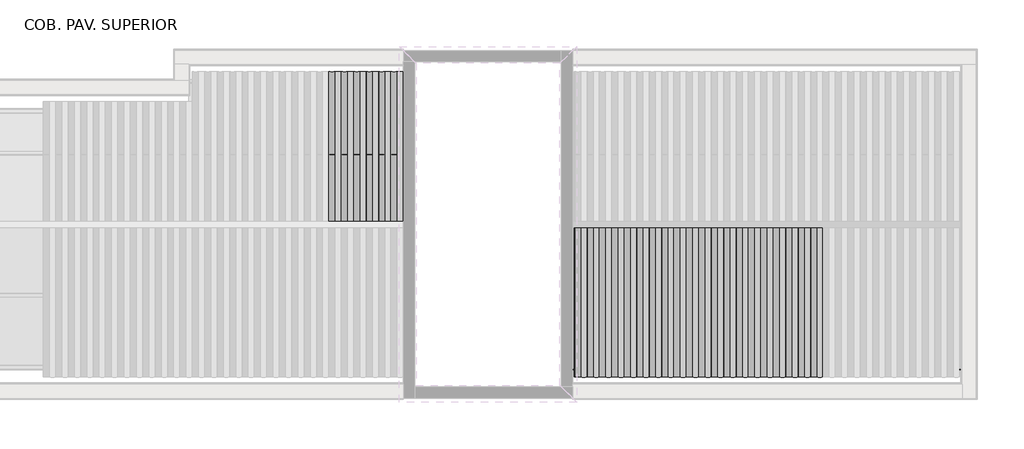
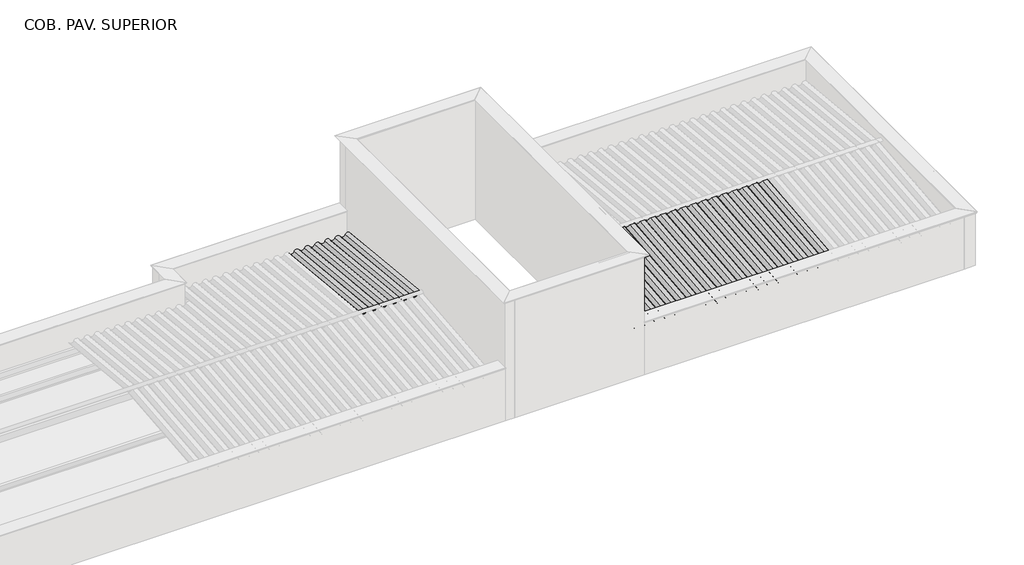
# One storey, part 5 of 7: 36 beams, 9 columns.
"""IFC4 building model written with IfcOpenShell, lengths in millimetres."""

import ifcopenshell
import ifcopenshell.guid

model = None  # the IFC model being written
_history = None  # IfcOwnerHistory: only IFC2X3 demands one
_inside = {}  # id of a spatial element -> (the spatial element, [elements in it])
_under = {}  # id of a project, library or spatial element -> (it, [spatial elements below it])
_declared = {}  # id of a project -> (the project, [libraries it declares])
_typed = {}  # id of a type object -> (the type object, [elements of that type])
_made_of = {}  # id of a material, layer set ... -> (it, [elements and type objects made of it])


def new_model(schema):
    """Start an empty IFC model of exactly this schema.

    Asked for "IFC4X3", IfcOpenShell would pick the latest addendum, in which some entities
    have other attributes; the version numbers below select the first issue.
    IFC2X3 requires an IfcOwnerHistory on every rooted entity: one is made here for all.
    """
    global model, _history
    if schema == "IFC4X3":
        model = ifcopenshell.file(schema_version=(4, 3, 0, 0))
    else:
        model = ifcopenshell.file(schema=schema)
    _inside.clear()
    _under.clear()
    _declared.clear()
    _typed.clear()
    _made_of.clear()
    _history = None
    if model.schema == "IFC2X3":
        org = make("IfcOrganization", Name="unknown")
        user = make(
            "IfcPersonAndOrganization",
            ThePerson=make("IfcPerson", FamilyName="unknown"),
            TheOrganization=org,
        )
        app = make(
            "IfcApplication",
            ApplicationDeveloper=org,
            Version="unknown",
            ApplicationFullName="unknown",
            ApplicationIdentifier="unknown",
        )
        _history = make(
            "IfcOwnerHistory",
            OwningUser=user,
            OwningApplication=app,
            ChangeAction="ADDED",
            CreationDate=0,
        )
    return model


def make(cls, **values):
    """One entity of the class cls with the attributes given. An attribute that is None is left unset."""
    return model.create_entity(
        cls, **{name: value for name, value in values.items() if value is not None}
    )


def rooted(cls, **values):
    """An entity with a GlobalId (a new one), such as an element, a storey or a relation."""
    return make(cls, GlobalId=ifcopenshell.guid.new(), OwnerHistory=_history, **values)


def si_unit(unit_type, name, prefix=None):
    """IfcSIUnit, for example si_unit("LENGTHUNIT", "METRE", prefix="MILLI")."""
    return make("IfcSIUnit", UnitType=unit_type, Prefix=prefix, Name=name)


def assignment(units):
    """IfcUnitAssignment: the units of a project."""
    return None if units is None else make("IfcUnitAssignment", Units=units)


def point(xyz):
    """IfcCartesianPoint."""
    return None if xyz is None else make("IfcCartesianPoint", Coordinates=xyz)


def direction(xyz):
    """IfcDirection."""
    return None if xyz is None else make("IfcDirection", DirectionRatios=xyz)


def frame(location, z_axis=None, x_axis=None):
    """IfcAxis2Placement3D, a coordinate frame: its origin and axes. An axis left out is left unset."""
    return make(
        "IfcAxis2Placement3D",
        Location=point(location),
        Axis=direction(z_axis),
        RefDirection=direction(x_axis),
    )


def frame_2d(location, x_axis=None):
    """IfcAxis2Placement2D, a coordinate frame in the plane: its origin and x axis."""
    return make(
        "IfcAxis2Placement2D", Location=point(location), RefDirection=direction(x_axis)
    )


def origin():
    """The frame at (0, 0, 0) with its axes left unset."""
    return frame((0.0, 0.0, 0.0))


def place(relative_to, where):
    """IfcLocalPlacement: puts the frame where relative to a parent placement (None: the world)."""
    return make(
        "IfcLocalPlacement", PlacementRelTo=relative_to, RelativePlacement=where
    )


def context(
    kind, dimensions, precision=None, world=None, true_north=None, identifier=None
):
    """IfcGeometricRepresentationContext, for example the 3D "Model" context."""
    return make(
        "IfcGeometricRepresentationContext",
        ContextIdentifier=identifier,
        ContextType=kind,
        CoordinateSpaceDimension=dimensions,
        Precision=precision,
        WorldCoordinateSystem=world,
        TrueNorth=true_north,
    )


def project(units=None, contexts=None):
    """IfcProject with its units and contexts."""
    return rooted(
        "IfcProject",
        Name="project",
        RepresentationContexts=contexts,
        UnitsInContext=assignment(units),
    )


def spatial(cls, under=None, at=None, **own):
    """A site, building, storey or space (cls), placed at a placement, below another one or the project."""
    s = rooted(cls, ObjectPlacement=at, **own)
    if under is not None:
        _under.setdefault(under.id(), (under, []))[1].append(s)
    return s


def polyline(points):
    """IfcPolyline through the points."""
    return make("IfcPolyline", Points=[point(p) for p in points])


def circle_curve(where, radius):
    """IfcCircle in the frame where."""
    return make("IfcCircle", Position=where, Radius=radius)


def trimmed(basis, trim1, trim2, sense, master):
    """IfcTrimmedCurve: the piece of a basis curve between two trims."""
    return make(
        "IfcTrimmedCurve",
        BasisCurve=basis,
        Trim1=trim1,
        Trim2=trim2,
        SenseAgreement=sense,
        MasterRepresentation=master,
    )


def segment(curve, same_sense, transition):
    """IfcCompositeCurveSegment."""
    return make(
        "IfcCompositeCurveSegment",
        Transition=transition,
        SameSense=same_sense,
        ParentCurve=curve,
    )


def composite_curve(segments, self_intersect=None):
    """IfcCompositeCurve: segments joined end to end."""
    return make("IfcCompositeCurve", Segments=segments, SelfIntersect=self_intersect)


def outline(outer, holes=None, kind="AREA"):
    """IfcArbitraryClosedProfileDef: a profile drawn as a closed curve; with holes, ...WithVoids."""
    if holes is None:
        return make("IfcArbitraryClosedProfileDef", ProfileType=kind, OuterCurve=outer)
    return make(
        "IfcArbitraryProfileDefWithVoids",
        ProfileType=kind,
        OuterCurve=outer,
        InnerCurves=holes,
    )


def extrude(swept, where, along, depth):
    """IfcExtrudedAreaSolid: the profile swept, set in the frame where, extruded along a direction by depth."""
    return make(
        "IfcExtrudedAreaSolid",
        SweptArea=swept,
        Position=where,
        ExtrudedDirection=direction(along),
        Depth=depth,
    )


def shape(context_of_items, identifier, shape_type, items):
    """IfcShapeRepresentation: the items that make up one representation, for example the "Body"."""
    return make(
        "IfcShapeRepresentation",
        ContextOfItems=context_of_items,
        RepresentationIdentifier=identifier,
        RepresentationType=shape_type,
        Items=items,
    )


def source(mapping_origin, context_of_items, identifier, shape_type, items):
    """IfcRepresentationMap: a shape defined once, which mapped items show again and again."""
    return make(
        "IfcRepresentationMap",
        MappingOrigin=mapping_origin,
        MappedRepresentation=shape(context_of_items, identifier, shape_type, items),
    )


def transform(
    local_origin,
    x_axis=None,
    y_axis=None,
    z_axis=None,
    scale=None,
    scale2=None,
    scale3=None,
    uniform=True,
):
    """IfcCartesianTransformationOperator3D, or its non-uniform kind. x_axis, y_axis, z_axis: its Axis1, 2, 3."""
    if uniform:
        return make(
            "IfcCartesianTransformationOperator3D",
            Axis1=direction(x_axis),
            Axis2=direction(y_axis),
            LocalOrigin=point(local_origin),
            Scale=scale,
            Axis3=direction(z_axis),
        )
    return make(
        "IfcCartesianTransformationOperator3DnonUniform",
        Axis1=direction(x_axis),
        Axis2=direction(y_axis),
        LocalOrigin=point(local_origin),
        Scale=scale,
        Axis3=direction(z_axis),
        Scale2=scale2,
        Scale3=scale3,
    )


def mapped(mapping_source, mapping_target):
    """IfcMappedItem: shows the shape of a source again, moved by a transform."""
    return make(
        "IfcMappedItem", MappingSource=mapping_source, MappingTarget=mapping_target
    )


def made_of(thing, what):
    """Note that an element or type object is made of a material, layer set ...; save() writes the relation."""
    if what is not None:
        _made_of.setdefault(what.id(), (what, []))[1].append(thing)
    return thing


def element(
    cls,
    number,
    at=None,
    inside=None,
    cuts=None,
    type_object=None,
    material=None,
    context=None,
    identifier="Body",
    shape_type=None,
    held_by="IfcProductDefinitionShape",
    body=None,
    shapes=None,
    **own,
):
    """One element of the class cls, such as IfcWall. Its Tag is "e" and its number.

    at: its placement. inside: the storey or other place that contains it. cuts: it is an
    opening in that element (IfcRelVoidsElement). A single representation is given by context,
    identifier, shape_type and body (its items); several are given by shapes. held_by: the class
    of the entity that holds the representations. save() writes the other relations.
    """
    e = rooted(cls, Tag="e%d" % number, ObjectPlacement=at, **own)
    if body is not None:
        shapes = [shape(context, identifier, shape_type, body)]
    if shapes is not None:
        e.Representation = make(held_by, Representations=shapes)
    if inside is not None:
        _inside.setdefault(inside.id(), (inside, []))[1].append(e)
    if cuts is not None:
        rooted(
            "IfcRelVoidsElement", RelatingBuildingElement=cuts, RelatedOpeningElement=e
        )
    if type_object is not None:
        _typed.setdefault(type_object.id(), (type_object, []))[1].append(e)
    return made_of(e, material)


def aggregate(whole, parts):
    """IfcRelAggregates: a whole, such as a stair, and the parts it consists of."""
    return rooted("IfcRelAggregates", RelatingObject=whole, RelatedObjects=parts)


def save(model, path):
    """Write the relations noted so far, then the file.

    IfcRelAggregates (storeys below a building ...), IfcRelContainedInSpatialStructure (elements
    in a storey), IfcRelDefinesByType, IfcRelAssociatesMaterial and IfcRelDeclares: one each for
    every whole, place, type object, material and project.
    """
    for whole, parts in _under.values():
        aggregate(whole, parts)
    for where, things in _inside.values():
        rooted(
            "IfcRelContainedInSpatialStructure",
            RelatedElements=things,
            RelatingStructure=where,
        )
    for kind, things in _typed.values():
        rooted("IfcRelDefinesByType", RelatedObjects=things, RelatingType=kind)
    for what, things in _made_of.values():
        rooted("IfcRelAssociatesMaterial", RelatedObjects=things, RelatingMaterial=what)
    for by, libraries in _declared.values():
        rooted("IfcRelDeclares", RelatingContext=by, RelatedDefinitions=libraries)
    model.write(path)


def column_4db371bd(model_context):
    return source(origin(), model_context, "Body", "SweptSolid", [
        extrude(outline(polyline([(30.0, 80.0), (30.0, -80.0), (-30.0, -80.0), (-30.0, 80.0), (30.0, 80.0)])), frame((0.0, 0.0, 6710.0), z_axis=(0.0, 0.0, 1.0), x_axis=(1.0, 0.0, 0.0)), (0.0, 0.0, 1.0), 660.0),
    ])


def column_e8b88e91(model_context):
    return source(origin(), model_context, "Body", "SweptSolid", [
        extrude(outline(polyline([(30.0, 80.0), (30.0, -80.0), (-30.0, -80.0), (-30.0, 80.0), (30.0, 80.0)])), frame((0.0, 0.0, 6710.0), z_axis=(0.0, 0.0, 1.0), x_axis=(1.0, 0.0, 0.0)), (0.0, 0.0, 1.0), 515.0),
    ])


def column_d0cf395a(model_context):
    return source(origin(), model_context, "Body", "SweptSolid", [
        extrude(outline(polyline([(30.0, 80.0), (30.0, -80.0), (-30.0, -80.0), (-30.0, 80.0), (30.0, 80.0)])), frame((0.0, 0.0, 6710.0), z_axis=(0.0, 0.0, 1.0), x_axis=(1.0, 0.0, 0.0)), (0.0, 0.0, 1.0), 520.0),
    ])


model = new_model("IFC4")

# Units and contexts
model_context = context("Model", 3, world=origin())
ifc_project = project(units=[si_unit("LENGTHUNIT", "METRE", prefix="MILLI")], contexts=[model_context])

# Site, building, storey
site = spatial("IfcSite", under=ifc_project)
building = spatial("IfcBuilding", under=site)
storey = spatial("IfcBuildingStorey", under=building, Name="COB. PAV. SUPERIOR", Elevation=6650.0)

# Beams
placement = place(None, origin())
element("IfcBeam", 1, ObjectType="Madeira de lei : Berço 6x12cm", at=placement, inside=storey, context=model_context, shape_type="SweptSolid", body=[
    extrude(outline(polyline([(-679.2813076, -6319.8711004), (-679.2813076, -6439.8711004), (-2679.2813064, -6439.8711004), (-2679.2813064, -6319.8711004), (-679.2813076, -6319.8711004)])), frame((0.0, 0.0, 6650.0), z_axis=(0.0, 0.0, 1.0), x_axis=(1.0, 0.0, 0.0)), (0.0, 0.0, 1.0), 60.0),
])
element("IfcBeam", 2, ObjectType="Madeira de lei : Berço 6x12cm", at=placement, inside=storey, context=model_context, shape_type="SweptSolid", body=[
    extrude(outline(polyline([(-259.281307, -6319.8711004), (-259.281307, -6439.8711004), (-679.2813064, -6439.8711004), (-679.2813064, -6319.8711004), (-259.281307, -6319.8711004)])), frame((0.0, 0.0, 6650.0), z_axis=(0.0, 0.0, 1.0), x_axis=(1.0, 0.0, 0.0)), (0.0, 0.0, 1.0), 60.0),
])
element("IfcBeam", 3, ObjectType="Madeira de lei : Berço 6x12cm", at=placement, inside=storey, context=model_context, shape_type="SweptSolid", body=[
    extrude(outline(polyline([(5089.718693, -9101.268869), (5089.718693, -9221.268869), (3089.718693, -9221.268869), (3089.718693, -9101.268869), (5089.718693, -9101.268869)])), frame((0.0, 0.0, 6650.0), z_axis=(0.0, 0.0, 1.0), x_axis=(1.0, 0.0, 0.0)), (0.0, 0.0, 1.0), 60.0),
])
element("IfcBeam", 4, ObjectType="Madeira de lei : Berço 6x12cm", at=placement, inside=storey, context=model_context, shape_type="SweptSolid", body=[
    extrude(outline(polyline([(5089.718693, -10521.818869), (5089.718693, -10641.818869), (3089.718693, -10641.818869), (3089.718693, -10521.818869), (5089.718693, -10521.818869)])), frame((0.0, 0.0, 6650.0), z_axis=(0.0, 0.0, 1.0), x_axis=(1.0, 0.0, 0.0)), (0.0, 0.0, 1.0), 60.0),
])
element("IfcBeam", 5, ObjectType="Madeira de lei : Berço 6x12cm", at=placement, inside=storey, context=model_context, shape_type="SweptSolid", body=[
    extrude(outline(polyline([(7089.718693, -9101.268869), (7089.718693, -9221.268869), (5089.718693, -9221.268869), (5089.718693, -9101.268869), (7089.718693, -9101.268869)])), frame((0.0, 0.0, 6650.0), z_axis=(0.0, 0.0, 1.0), x_axis=(1.0, 0.0, 0.0)), (0.0, 0.0, 1.0), 60.0),
])
element("IfcBeam", 6, ObjectType="Madeira de lei : Berço 6x12cm", at=placement, inside=storey, context=model_context, shape_type="SweptSolid", body=[
    extrude(outline(polyline([(7089.718693, -10521.818869), (7089.718693, -10641.818869), (5089.718693, -10641.818869), (5089.718693, -10521.818869), (7089.718693, -10521.818869)])), frame((0.0, 0.0, 6650.0), z_axis=(0.0, 0.0, 1.0), x_axis=(1.0, 0.0, 0.0)), (0.0, 0.0, 1.0), 60.0),
])
element("IfcBeam", 7, ObjectType="Madeira de lei : Berço 6x12cm", at=placement, inside=storey, context=model_context, shape_type="SweptSolid", body=[
    extrude(outline(polyline([(9089.718693, -10521.818869), (9089.718693, -10641.818869), (7089.718693, -10641.818869), (7089.718693, -10521.818869), (9089.718693, -10521.818869)])), frame((0.0, 0.0, 6650.0), z_axis=(0.0, 0.0, 1.0), x_axis=(1.0, 0.0, 0.0)), (0.0, 0.0, 1.0), 60.0),
])
element("IfcBeam", 8, ObjectType="Madeira de lei : Berço 6x12cm", at=placement, inside=storey, context=model_context, shape_type="SweptSolid", body=[
    extrude(outline(polyline([(10729.718693, -10521.818869), (10729.718693, -10641.818869), (9089.718693, -10641.818869), (9089.718693, -10521.818869), (10729.718693, -10521.818869)])), frame((0.0, 0.0, 6650.0), z_axis=(0.0, 0.0, 1.0), x_axis=(1.0, 0.0, 0.0)), (0.0, 0.0, 1.0), 60.0),
])
element("IfcBeam", 9, ObjectType="Madeira de lei : Berço 6x12cm", at=placement, inside=storey, context=model_context, shape_type="SweptSolid", body=[
    extrude(outline(polyline([(-270.281307, -4899.3026908), (-270.281307, -5019.3026908), (-2270.2813064, -5019.3026908), (-2270.2813064, -4899.3026908), (-270.281307, -4899.3026908)])), frame((0.0, 0.0, 6650.0), z_axis=(0.0, 0.0, 1.0), x_axis=(1.0, 0.0, 0.0)), (0.0, 0.0, 1.0), 60.0),
])
element("IfcBeam", 10, ObjectType="Madeira de lei : Berço 6x12cm", at=placement, inside=storey, context=model_context, shape_type="SweptSolid", body=[
    extrude(outline(polyline([(-2270.2813076, -4899.3026908), (-2270.2813076, -5019.3026908), (-4270.281307, -5019.3026908), (-4270.281307, -4899.3026908), (-2270.2813076, -4899.3026908)])), frame((0.0, 0.0, 6650.0), z_axis=(0.0, 0.0, 1.0), x_axis=(1.0, 0.0, 0.0)), (0.0, 0.0, 1.0), 60.0),
])
element("IfcBeam", 11, ObjectType="Telha Ondulada : Fibrocimento", at=placement, inside=storey, context=model_context, shape_type="SweptSolid", body=[
    extrude(outline(composite_curve([segment(trimmed(circle_curve(frame_2d((0.0, 66.7939461)), 66.7939461), [point((29.3501489, 6.7939461))], [point((29.3501489, 126.7939461))], True, "CARTESIAN"), True, "CONTINUOUS"), segment(polyline([(29.3501489, 126.7939461), (31.5472154, 131.2853711)]), True, "CONTINUOUS"), segment(trimmed(circle_curve(frame_2d((0.0, 66.7939461)), 71.7939461), [point((31.5472154, 131.2853711))], [point((31.5472154, 2.3025211))], False, "CARTESIAN"), True, "CONTINUOUS"), segment(trimmed(circle_curve(frame_2d((58.7002978, -53.2060539)), 61.7939461), [point((31.5472154, 2.3025211))], [point((31.5472154, -108.7146289))], True, "CARTESIAN"), True, "CONTINUOUS"), segment(polyline([(31.5472154, -108.7146289), (29.3501489, -113.2060539)]), True, "CONTINUOUS"), segment(trimmed(circle_curve(frame_2d((58.7002978, -53.2060539)), 66.7939461), [point((29.3501489, -113.2060539))], [point((29.3501489, 6.7939461))], False, "CARTESIAN"), True, "CONTINUOUS")], self_intersect=False)), frame((3256.1156257, -10781.9594023, 7394.5315886), z_axis=(0.0, 0.9950371902099894, 0.09950371902099751), x_axis=(0.0, 0.09950371902099751, -0.9950371902099894)), (0.0, 0.0, 1.0), 3017.2387654),
])
element("IfcBeam", 12, ObjectType="Telha Ondulada : Fibrocimento", at=placement, inside=storey, context=model_context, shape_type="SweptSolid", body=[
    extrude(outline(composite_curve([segment(trimmed(circle_curve(frame_2d((0.0, 66.7939461)), 66.7939461), [point((29.3501489, 6.7939461))], [point((29.3501489, 126.7939461))], True, "CARTESIAN"), True, "CONTINUOUS"), segment(polyline([(29.3501489, 126.7939461), (31.5472154, 131.2853711)]), True, "CONTINUOUS"), segment(trimmed(circle_curve(frame_2d((0.0, 66.7939461)), 71.7939461), [point((31.5472154, 131.2853711))], [point((31.5472154, 2.3025211))], False, "CARTESIAN"), True, "CONTINUOUS"), segment(trimmed(circle_curve(frame_2d((58.7002978, -53.2060539)), 61.7939461), [point((31.5472154, 2.3025211))], [point((31.5472154, -108.7146289))], True, "CARTESIAN"), True, "CONTINUOUS"), segment(polyline([(31.5472154, -108.7146289), (29.3501489, -113.2060539)]), True, "CONTINUOUS"), segment(trimmed(circle_curve(frame_2d((58.7002978, -53.2060539)), 66.7939461), [point((29.3501489, -113.2060539))], [point((29.3501489, 6.7939461))], False, "CARTESIAN"), True, "CONTINUOUS")], self_intersect=False)), frame((3500.6156257, -10781.9594023, 7394.5315886), z_axis=(0.0, 0.9950371902099894, 0.09950371902099751), x_axis=(0.0, 0.09950371902099751, -0.9950371902099894)), (0.0, 0.0, 1.0), 3017.2387654),
])
element("IfcBeam", 13, ObjectType="Telha Ondulada : Fibrocimento", at=placement, inside=storey, context=model_context, shape_type="SweptSolid", body=[
    extrude(outline(composite_curve([segment(trimmed(circle_curve(frame_2d((0.0, 66.7939461)), 66.7939461), [point((29.3501489, 6.7939461))], [point((29.3501489, 126.7939461))], True, "CARTESIAN"), True, "CONTINUOUS"), segment(polyline([(29.3501489, 126.7939461), (31.5472154, 131.2853711)]), True, "CONTINUOUS"), segment(trimmed(circle_curve(frame_2d((0.0, 66.7939461)), 71.7939461), [point((31.5472154, 131.2853711))], [point((31.5472154, 2.3025211))], False, "CARTESIAN"), True, "CONTINUOUS"), segment(trimmed(circle_curve(frame_2d((58.7002978, -53.2060539)), 61.7939461), [point((31.5472154, 2.3025211))], [point((31.5472154, -108.7146289))], True, "CARTESIAN"), True, "CONTINUOUS"), segment(polyline([(31.5472154, -108.7146289), (29.3501489, -113.2060539)]), True, "CONTINUOUS"), segment(trimmed(circle_curve(frame_2d((58.7002978, -53.2060539)), 66.7939461), [point((29.3501489, -113.2060539))], [point((29.3501489, 6.7939461))], False, "CARTESIAN"), True, "CONTINUOUS")], self_intersect=False)), frame((3745.1156257, -10781.9594023, 7394.5315886), z_axis=(0.0, 0.9950371902099894, 0.09950371902099751), x_axis=(0.0, 0.09950371902099751, -0.9950371902099894)), (0.0, 0.0, 1.0), 3017.2387654),
])
element("IfcBeam", 14, ObjectType="Telha Ondulada : Fibrocimento", at=placement, inside=storey, context=model_context, shape_type="SweptSolid", body=[
    extrude(outline(composite_curve([segment(trimmed(circle_curve(frame_2d((0.0, 66.7939461)), 66.7939461), [point((29.3501489, 6.7939461))], [point((29.3501489, 126.7939461))], True, "CARTESIAN"), True, "CONTINUOUS"), segment(polyline([(29.3501489, 126.7939461), (31.5472154, 131.2853711)]), True, "CONTINUOUS"), segment(trimmed(circle_curve(frame_2d((0.0, 66.7939461)), 71.7939461), [point((31.5472154, 131.2853711))], [point((31.5472154, 2.3025211))], False, "CARTESIAN"), True, "CONTINUOUS"), segment(trimmed(circle_curve(frame_2d((58.7002978, -53.2060539)), 61.7939461), [point((31.5472154, 2.3025211))], [point((31.5472154, -108.7146289))], True, "CARTESIAN"), True, "CONTINUOUS"), segment(polyline([(31.5472154, -108.7146289), (29.3501489, -113.2060539)]), True, "CONTINUOUS"), segment(trimmed(circle_curve(frame_2d((58.7002978, -53.2060539)), 66.7939461), [point((29.3501489, -113.2060539))], [point((29.3501489, 6.7939461))], False, "CARTESIAN"), True, "CONTINUOUS")], self_intersect=False)), frame((3989.6156257, -10781.9594023, 7394.5315886), z_axis=(0.0, 0.9950371902099894, 0.09950371902099747), x_axis=(0.0, 0.09950371902099747, -0.9950371902099894)), (0.0, 0.0, 1.0), 3017.2387654),
])
element("IfcBeam", 15, ObjectType="Telha Ondulada : Fibrocimento", at=placement, inside=storey, context=model_context, shape_type="SweptSolid", body=[
    extrude(outline(composite_curve([segment(trimmed(circle_curve(frame_2d((0.0, 66.7939461)), 66.7939461), [point((29.3501489, 6.7939461))], [point((29.3501489, 126.7939461))], True, "CARTESIAN"), True, "CONTINUOUS"), segment(polyline([(29.3501489, 126.7939461), (31.5472154, 131.2853711)]), True, "CONTINUOUS"), segment(trimmed(circle_curve(frame_2d((0.0, 66.7939461)), 71.7939461), [point((31.5472154, 131.2853711))], [point((31.5472154, 2.3025211))], False, "CARTESIAN"), True, "CONTINUOUS"), segment(trimmed(circle_curve(frame_2d((58.7002978, -53.2060539)), 61.7939461), [point((31.5472154, 2.3025211))], [point((31.5472154, -108.7146289))], True, "CARTESIAN"), True, "CONTINUOUS"), segment(polyline([(31.5472154, -108.7146289), (29.3501489, -113.2060539)]), True, "CONTINUOUS"), segment(trimmed(circle_curve(frame_2d((58.7002978, -53.2060539)), 66.7939461), [point((29.3501489, -113.2060539))], [point((29.3501489, 6.7939461))], False, "CARTESIAN"), True, "CONTINUOUS")], self_intersect=False)), frame((4234.1156257, -10781.9594023, 7394.5315886), z_axis=(0.0, 0.9950371902099894, 0.09950371902099747), x_axis=(0.0, 0.09950371902099747, -0.9950371902099894)), (0.0, 0.0, 1.0), 3017.2387654),
])
element("IfcBeam", 16, ObjectType="Telha Ondulada : Fibrocimento", at=placement, inside=storey, context=model_context, shape_type="SweptSolid", body=[
    extrude(outline(composite_curve([segment(trimmed(circle_curve(frame_2d((0.0, 66.7939461)), 66.7939461), [point((29.3501489, 6.7939461))], [point((29.3501489, 126.7939461))], True, "CARTESIAN"), True, "CONTINUOUS"), segment(polyline([(29.3501489, 126.7939461), (31.5472154, 131.2853711)]), True, "CONTINUOUS"), segment(trimmed(circle_curve(frame_2d((0.0, 66.7939461)), 71.7939461), [point((31.5472154, 131.2853711))], [point((31.5472154, 2.3025211))], False, "CARTESIAN"), True, "CONTINUOUS"), segment(trimmed(circle_curve(frame_2d((58.7002978, -53.2060539)), 61.7939461), [point((31.5472154, 2.3025211))], [point((31.5472154, -108.7146289))], True, "CARTESIAN"), True, "CONTINUOUS"), segment(polyline([(31.5472154, -108.7146289), (29.3501489, -113.2060539)]), True, "CONTINUOUS"), segment(trimmed(circle_curve(frame_2d((58.7002978, -53.2060539)), 66.7939461), [point((29.3501489, -113.2060539))], [point((29.3501489, 6.7939461))], False, "CARTESIAN"), True, "CONTINUOUS")], self_intersect=False)), frame((4478.6156257, -10781.9594023, 7394.5315886), z_axis=(0.0, 0.9950371902099894, 0.09950371902099744), x_axis=(0.0, 0.09950371902099744, -0.9950371902099894)), (0.0, 0.0, 1.0), 3017.2387654),
])
element("IfcBeam", 17, ObjectType="Telha Ondulada : Fibrocimento", at=placement, inside=storey, context=model_context, shape_type="SweptSolid", body=[
    extrude(outline(composite_curve([segment(trimmed(circle_curve(frame_2d((0.0, 66.7939461)), 66.7939461), [point((29.3501489, 6.7939461))], [point((29.3501489, 126.7939461))], True, "CARTESIAN"), True, "CONTINUOUS"), segment(polyline([(29.3501489, 126.7939461), (31.5472154, 131.2853711)]), True, "CONTINUOUS"), segment(trimmed(circle_curve(frame_2d((0.0, 66.7939461)), 71.7939461), [point((31.5472154, 131.2853711))], [point((31.5472154, 2.3025211))], False, "CARTESIAN"), True, "CONTINUOUS"), segment(trimmed(circle_curve(frame_2d((58.7002978, -53.2060539)), 61.7939461), [point((31.5472154, 2.3025211))], [point((31.5472154, -108.7146289))], True, "CARTESIAN"), True, "CONTINUOUS"), segment(polyline([(31.5472154, -108.7146289), (29.3501489, -113.2060539)]), True, "CONTINUOUS"), segment(trimmed(circle_curve(frame_2d((58.7002978, -53.2060539)), 66.7939461), [point((29.3501489, -113.2060539))], [point((29.3501489, 6.7939461))], False, "CARTESIAN"), True, "CONTINUOUS")], self_intersect=False)), frame((4723.1156257, -10781.9594023, 7394.5315886), z_axis=(0.0, 0.9950371902099894, 0.09950371902099751), x_axis=(0.0, 0.09950371902099751, -0.9950371902099894)), (0.0, 0.0, 1.0), 3017.2387654),
])
element("IfcBeam", 18, ObjectType="Telha Ondulada : Fibrocimento", at=placement, inside=storey, context=model_context, shape_type="SweptSolid", body=[
    extrude(outline(composite_curve([segment(trimmed(circle_curve(frame_2d((0.0, 66.7939461)), 66.7939461), [point((29.3501489, 6.7939461))], [point((29.3501489, 126.7939461))], True, "CARTESIAN"), True, "CONTINUOUS"), segment(polyline([(29.3501489, 126.7939461), (31.5472154, 131.2853711)]), True, "CONTINUOUS"), segment(trimmed(circle_curve(frame_2d((0.0, 66.7939461)), 71.7939461), [point((31.5472154, 131.2853711))], [point((31.5472154, 2.3025211))], False, "CARTESIAN"), True, "CONTINUOUS"), segment(trimmed(circle_curve(frame_2d((58.7002978, -53.2060539)), 61.7939461), [point((31.5472154, 2.3025211))], [point((31.5472154, -108.7146289))], True, "CARTESIAN"), True, "CONTINUOUS"), segment(polyline([(31.5472154, -108.7146289), (29.3501489, -113.2060539)]), True, "CONTINUOUS"), segment(trimmed(circle_curve(frame_2d((58.7002978, -53.2060539)), 66.7939461), [point((29.3501489, -113.2060539))], [point((29.3501489, 6.7939461))], False, "CARTESIAN"), True, "CONTINUOUS")], self_intersect=False)), frame((4967.6156257, -10781.9594023, 7394.5315886), z_axis=(0.0, 0.9950371902099894, 0.09950371902099751), x_axis=(0.0, 0.09950371902099751, -0.9950371902099894)), (0.0, 0.0, 1.0), 3017.2387654),
])
element("IfcBeam", 19, ObjectType="Telha Ondulada : Fibrocimento", at=placement, inside=storey, context=model_context, shape_type="SweptSolid", body=[
    extrude(outline(composite_curve([segment(trimmed(circle_curve(frame_2d((0.0, 66.7939461)), 66.7939461), [point((29.3501489, 6.7939461))], [point((29.3501489, 126.7939461))], True, "CARTESIAN"), True, "CONTINUOUS"), segment(polyline([(29.3501489, 126.7939461), (31.5472154, 131.2853711)]), True, "CONTINUOUS"), segment(trimmed(circle_curve(frame_2d((0.0, 66.7939461)), 71.7939461), [point((31.5472154, 131.2853711))], [point((31.5472154, 2.3025211))], False, "CARTESIAN"), True, "CONTINUOUS"), segment(trimmed(circle_curve(frame_2d((58.7002978, -53.2060539)), 61.7939461), [point((31.5472154, 2.3025211))], [point((31.5472154, -108.7146289))], True, "CARTESIAN"), True, "CONTINUOUS"), segment(polyline([(31.5472154, -108.7146289), (29.3501489, -113.2060539)]), True, "CONTINUOUS"), segment(trimmed(circle_curve(frame_2d((58.7002978, -53.2060539)), 66.7939461), [point((29.3501489, -113.2060539))], [point((29.3501489, 6.7939461))], False, "CARTESIAN"), True, "CONTINUOUS")], self_intersect=False)), frame((5212.1156257, -10781.9594023, 7394.5315886), z_axis=(0.0, 0.9950371902099894, 0.09950371902099751), x_axis=(0.0, 0.09950371902099751, -0.9950371902099894)), (0.0, 0.0, 1.0), 3017.2387654),
])
element("IfcBeam", 20, ObjectType="Telha Ondulada : Fibrocimento", at=placement, inside=storey, context=model_context, shape_type="SweptSolid", body=[
    extrude(outline(composite_curve([segment(trimmed(circle_curve(frame_2d((0.0, 66.7939461)), 66.7939461), [point((29.3501489, 6.7939461))], [point((29.3501489, 126.7939461))], True, "CARTESIAN"), True, "CONTINUOUS"), segment(polyline([(29.3501489, 126.7939461), (31.5472154, 131.2853711)]), True, "CONTINUOUS"), segment(trimmed(circle_curve(frame_2d((0.0, 66.7939461)), 71.7939461), [point((31.5472154, 131.2853711))], [point((31.5472154, 2.3025211))], False, "CARTESIAN"), True, "CONTINUOUS"), segment(trimmed(circle_curve(frame_2d((58.7002978, -53.2060539)), 61.7939461), [point((31.5472154, 2.3025211))], [point((31.5472154, -108.7146289))], True, "CARTESIAN"), True, "CONTINUOUS"), segment(polyline([(31.5472154, -108.7146289), (29.3501489, -113.2060539)]), True, "CONTINUOUS"), segment(trimmed(circle_curve(frame_2d((58.7002978, -53.2060539)), 66.7939461), [point((29.3501489, -113.2060539))], [point((29.3501489, 6.7939461))], False, "CARTESIAN"), True, "CONTINUOUS")], self_intersect=False)), frame((5456.6156257, -10781.9594023, 7394.5315886), z_axis=(0.0, 0.9950371902099894, 0.09950371902099751), x_axis=(0.0, 0.09950371902099751, -0.9950371902099894)), (0.0, 0.0, 1.0), 3017.2387654),
])
element("IfcBeam", 21, ObjectType="Telha Ondulada : Fibrocimento", at=placement, inside=storey, context=model_context, shape_type="SweptSolid", body=[
    extrude(outline(composite_curve([segment(trimmed(circle_curve(frame_2d((0.0, 66.7939461)), 66.7939461), [point((29.3501489, 6.7939461))], [point((29.3501489, 126.7939461))], True, "CARTESIAN"), True, "CONTINUOUS"), segment(polyline([(29.3501489, 126.7939461), (31.5472154, 131.2853711)]), True, "CONTINUOUS"), segment(trimmed(circle_curve(frame_2d((0.0, 66.7939461)), 71.7939461), [point((31.5472154, 131.2853711))], [point((31.5472154, 2.3025211))], False, "CARTESIAN"), True, "CONTINUOUS"), segment(trimmed(circle_curve(frame_2d((58.7002978, -53.2060539)), 61.7939461), [point((31.5472154, 2.3025211))], [point((31.5472154, -108.7146289))], True, "CARTESIAN"), True, "CONTINUOUS"), segment(polyline([(31.5472154, -108.7146289), (29.3501489, -113.2060539)]), True, "CONTINUOUS"), segment(trimmed(circle_curve(frame_2d((58.7002978, -53.2060539)), 66.7939461), [point((29.3501489, -113.2060539))], [point((29.3501489, 6.7939461))], False, "CARTESIAN"), True, "CONTINUOUS")], self_intersect=False)), frame((5701.1156257, -10781.9594023, 7394.5315886), z_axis=(0.0, 0.9950371902099894, 0.09950371902099747), x_axis=(0.0, 0.09950371902099747, -0.9950371902099894)), (0.0, 0.0, 1.0), 3017.2387654),
])
element("IfcBeam", 22, ObjectType="Telha Ondulada : Fibrocimento", at=placement, inside=storey, context=model_context, shape_type="SweptSolid", body=[
    extrude(outline(composite_curve([segment(trimmed(circle_curve(frame_2d((0.0, 66.7939461)), 66.7939461), [point((29.3501489, 6.7939461))], [point((29.3501489, 126.7939461))], True, "CARTESIAN"), True, "CONTINUOUS"), segment(polyline([(29.3501489, 126.7939461), (31.5472154, 131.2853711)]), True, "CONTINUOUS"), segment(trimmed(circle_curve(frame_2d((0.0, 66.7939461)), 71.7939461), [point((31.5472154, 131.2853711))], [point((31.5472154, 2.3025211))], False, "CARTESIAN"), True, "CONTINUOUS"), segment(trimmed(circle_curve(frame_2d((58.7002978, -53.2060539)), 61.7939461), [point((31.5472154, 2.3025211))], [point((31.5472154, -108.7146289))], True, "CARTESIAN"), True, "CONTINUOUS"), segment(polyline([(31.5472154, -108.7146289), (29.3501489, -113.2060539)]), True, "CONTINUOUS"), segment(trimmed(circle_curve(frame_2d((58.7002978, -53.2060539)), 66.7939461), [point((29.3501489, -113.2060539))], [point((29.3501489, 6.7939461))], False, "CARTESIAN"), True, "CONTINUOUS")], self_intersect=False)), frame((5945.6156257, -10781.9594023, 7394.5315886), z_axis=(0.0, 0.9950371902099894, 0.09950371902099751), x_axis=(0.0, 0.09950371902099751, -0.9950371902099894)), (0.0, 0.0, 1.0), 3017.2387654),
])
element("IfcBeam", 23, ObjectType="Telha Ondulada : Fibrocimento", at=placement, inside=storey, context=model_context, shape_type="SweptSolid", body=[
    extrude(outline(composite_curve([segment(trimmed(circle_curve(frame_2d((0.0, 66.7939461)), 66.7939461), [point((29.3501489, 6.7939461))], [point((29.3501489, 126.7939461))], True, "CARTESIAN"), True, "CONTINUOUS"), segment(polyline([(29.3501489, 126.7939461), (31.5472154, 131.2853711)]), True, "CONTINUOUS"), segment(trimmed(circle_curve(frame_2d((0.0, 66.7939461)), 71.7939461), [point((31.5472154, 131.2853711))], [point((31.5472154, 2.3025211))], False, "CARTESIAN"), True, "CONTINUOUS"), segment(trimmed(circle_curve(frame_2d((58.7002978, -53.2060539)), 61.7939461), [point((31.5472154, 2.3025211))], [point((31.5472154, -108.7146289))], True, "CARTESIAN"), True, "CONTINUOUS"), segment(polyline([(31.5472154, -108.7146289), (29.3501489, -113.2060539)]), True, "CONTINUOUS"), segment(trimmed(circle_curve(frame_2d((58.7002978, -53.2060539)), 66.7939461), [point((29.3501489, -113.2060539))], [point((29.3501489, 6.7939461))], False, "CARTESIAN"), True, "CONTINUOUS")], self_intersect=False)), frame((6190.1156257, -10781.9594023, 7394.5315886), z_axis=(0.0, 0.9950371902099894, 0.09950371902099754), x_axis=(0.0, 0.09950371902099754, -0.9950371902099894)), (0.0, 0.0, 1.0), 3017.2387654),
])
element("IfcBeam", 24, ObjectType="Telha Ondulada : Fibrocimento", at=placement, inside=storey, context=model_context, shape_type="SweptSolid", body=[
    extrude(outline(composite_curve([segment(trimmed(circle_curve(frame_2d((0.0, 66.7939461)), 66.7939461), [point((29.3501489, 6.7939461))], [point((29.3501489, 126.7939461))], True, "CARTESIAN"), True, "CONTINUOUS"), segment(polyline([(29.3501489, 126.7939461), (31.5472154, 131.2853711)]), True, "CONTINUOUS"), segment(trimmed(circle_curve(frame_2d((0.0, 66.7939461)), 71.7939461), [point((31.5472154, 131.2853711))], [point((31.5472154, 2.3025211))], False, "CARTESIAN"), True, "CONTINUOUS"), segment(trimmed(circle_curve(frame_2d((58.7002978, -53.2060539)), 61.7939461), [point((31.5472154, 2.3025211))], [point((31.5472154, -108.7146289))], True, "CARTESIAN"), True, "CONTINUOUS"), segment(polyline([(31.5472154, -108.7146289), (29.3501489, -113.2060539)]), True, "CONTINUOUS"), segment(trimmed(circle_curve(frame_2d((58.7002978, -53.2060539)), 66.7939461), [point((29.3501489, -113.2060539))], [point((29.3501489, 6.7939461))], False, "CARTESIAN"), True, "CONTINUOUS")], self_intersect=False)), frame((6434.6156257, -10781.9594023, 7394.5315886), z_axis=(0.0, 0.9950371902099894, 0.09950371902099751), x_axis=(0.0, 0.09950371902099751, -0.9950371902099894)), (0.0, 0.0, 1.0), 3017.2387654),
])
element("IfcBeam", 25, ObjectType="Telha Ondulada : Fibrocimento", at=placement, inside=storey, context=model_context, shape_type="SweptSolid", body=[
    extrude(outline(composite_curve([segment(trimmed(circle_curve(frame_2d((0.0, 66.7939461)), 66.7939461), [point((29.3501489, 6.7939461))], [point((29.3501489, 126.7939461))], True, "CARTESIAN"), True, "CONTINUOUS"), segment(polyline([(29.3501489, 126.7939461), (31.5472154, 131.2853711)]), True, "CONTINUOUS"), segment(trimmed(circle_curve(frame_2d((0.0, 66.7939461)), 71.7939461), [point((31.5472154, 131.2853711))], [point((31.5472154, 2.3025211))], False, "CARTESIAN"), True, "CONTINUOUS"), segment(trimmed(circle_curve(frame_2d((58.7002978, -53.2060539)), 61.7939461), [point((31.5472154, 2.3025211))], [point((31.5472154, -108.7146289))], True, "CARTESIAN"), True, "CONTINUOUS"), segment(polyline([(31.5472154, -108.7146289), (29.3501489, -113.2060539)]), True, "CONTINUOUS"), segment(trimmed(circle_curve(frame_2d((58.7002978, -53.2060539)), 66.7939461), [point((29.3501489, -113.2060539))], [point((29.3501489, 6.7939461))], False, "CARTESIAN"), True, "CONTINUOUS")], self_intersect=False)), frame((6679.1156257, -10781.9594023, 7394.5315886), z_axis=(0.0, 0.9950371902099894, 0.09950371902099751), x_axis=(0.0, 0.09950371902099751, -0.9950371902099894)), (0.0, 0.0, 1.0), 3017.2387654),
])
element("IfcBeam", 26, ObjectType="Telha Ondulada : Fibrocimento", at=placement, inside=storey, context=model_context, shape_type="SweptSolid", body=[
    extrude(outline(composite_curve([segment(trimmed(circle_curve(frame_2d((0.0, 66.7939461)), 66.7939461), [point((29.3501489, 6.7939461))], [point((29.3501489, 126.7939461))], True, "CARTESIAN"), True, "CONTINUOUS"), segment(polyline([(29.3501489, 126.7939461), (31.5472154, 131.2853711)]), True, "CONTINUOUS"), segment(trimmed(circle_curve(frame_2d((0.0, 66.7939461)), 71.7939461), [point((31.5472154, 131.2853711))], [point((31.5472154, 2.3025211))], False, "CARTESIAN"), True, "CONTINUOUS"), segment(trimmed(circle_curve(frame_2d((58.7002978, -53.2060539)), 61.7939461), [point((31.5472154, 2.3025211))], [point((31.5472154, -108.7146289))], True, "CARTESIAN"), True, "CONTINUOUS"), segment(polyline([(31.5472154, -108.7146289), (29.3501489, -113.2060539)]), True, "CONTINUOUS"), segment(trimmed(circle_curve(frame_2d((58.7002978, -53.2060539)), 66.7939461), [point((29.3501489, -113.2060539))], [point((29.3501489, 6.7939461))], False, "CARTESIAN"), True, "CONTINUOUS")], self_intersect=False)), frame((6923.6156257, -10781.9594023, 7394.5315886), z_axis=(0.0, 0.9950371902099894, 0.09950371902099751), x_axis=(0.0, 0.09950371902099751, -0.9950371902099894)), (0.0, 0.0, 1.0), 3017.2387654),
])
element("IfcBeam", 27, ObjectType="Telha Ondulada : Fibrocimento", at=placement, inside=storey, context=model_context, shape_type="SweptSolid", body=[
    extrude(outline(composite_curve([segment(trimmed(circle_curve(frame_2d((0.0, 66.7939461)), 66.7939461), [point((29.3501489, 6.7939461))], [point((29.3501489, 126.7939461))], True, "CARTESIAN"), True, "CONTINUOUS"), segment(polyline([(29.3501489, 126.7939461), (31.5472154, 131.2853711)]), True, "CONTINUOUS"), segment(trimmed(circle_curve(frame_2d((0.0, 66.7939461)), 71.7939461), [point((31.5472154, 131.2853711))], [point((31.5472154, 2.3025211))], False, "CARTESIAN"), True, "CONTINUOUS"), segment(trimmed(circle_curve(frame_2d((58.7002978, -53.2060539)), 61.7939461), [point((31.5472154, 2.3025211))], [point((31.5472154, -108.7146289))], True, "CARTESIAN"), True, "CONTINUOUS"), segment(polyline([(31.5472154, -108.7146289), (29.3501489, -113.2060539)]), True, "CONTINUOUS"), segment(trimmed(circle_curve(frame_2d((58.7002978, -53.2060539)), 66.7939461), [point((29.3501489, -113.2060539))], [point((29.3501489, 6.7939461))], False, "CARTESIAN"), True, "CONTINUOUS")], self_intersect=False)), frame((7168.1156257, -10781.9594023, 7394.5315886), z_axis=(0.0, 0.9950371902099894, 0.09950371902099751), x_axis=(0.0, 0.09950371902099751, -0.9950371902099894)), (0.0, 0.0, 1.0), 3017.2387654),
])
element("IfcBeam", 28, ObjectType="Telha Ondulada : Fibrocimento", at=placement, inside=storey, context=model_context, shape_type="SweptSolid", body=[
    extrude(outline(composite_curve([segment(trimmed(circle_curve(frame_2d((0.0, 66.7939461)), 66.7939461), [point((29.3501489, 6.7939461))], [point((29.3501489, 126.7939461))], True, "CARTESIAN"), True, "CONTINUOUS"), segment(polyline([(29.3501489, 126.7939461), (31.5472154, 131.2853711)]), True, "CONTINUOUS"), segment(trimmed(circle_curve(frame_2d((0.0, 66.7939461)), 71.7939461), [point((31.5472154, 131.2853711))], [point((31.5472154, 2.3025211))], False, "CARTESIAN"), True, "CONTINUOUS"), segment(trimmed(circle_curve(frame_2d((58.7002978, -53.2060539)), 61.7939461), [point((31.5472154, 2.3025211))], [point((31.5472154, -108.7146289))], True, "CARTESIAN"), True, "CONTINUOUS"), segment(polyline([(31.5472154, -108.7146289), (29.3501489, -113.2060539)]), True, "CONTINUOUS"), segment(trimmed(circle_curve(frame_2d((58.7002978, -53.2060539)), 66.7939461), [point((29.3501489, -113.2060539))], [point((29.3501489, 6.7939461))], False, "CARTESIAN"), True, "CONTINUOUS")], self_intersect=False)), frame((7412.6156257, -10781.9594023, 7394.5315886), z_axis=(0.0, 0.9950371902099894, 0.09950371902099747), x_axis=(0.0, 0.09950371902099747, -0.9950371902099894)), (0.0, 0.0, 1.0), 3017.2387654),
])
element("IfcBeam", 29, ObjectType="Telha Ondulada : Fibrocimento", at=placement, inside=storey, context=model_context, shape_type="SweptSolid", body=[
    extrude(outline(composite_curve([segment(trimmed(circle_curve(frame_2d((0.0, 66.7939461)), 66.7939461), [point((29.3501489, 6.7939461))], [point((29.3501489, 126.7939461))], True, "CARTESIAN"), True, "CONTINUOUS"), segment(polyline([(29.3501489, 126.7939461), (31.5472154, 131.2853711)]), True, "CONTINUOUS"), segment(trimmed(circle_curve(frame_2d((0.0, 66.7939461)), 71.7939461), [point((31.5472154, 131.2853711))], [point((31.5472154, 2.3025211))], False, "CARTESIAN"), True, "CONTINUOUS"), segment(trimmed(circle_curve(frame_2d((58.7002978, -53.2060539)), 61.7939461), [point((31.5472154, 2.3025211))], [point((31.5472154, -108.7146289))], True, "CARTESIAN"), True, "CONTINUOUS"), segment(polyline([(31.5472154, -108.7146289), (29.3501489, -113.2060539)]), True, "CONTINUOUS"), segment(trimmed(circle_curve(frame_2d((58.7002978, -53.2060539)), 66.7939461), [point((29.3501489, -113.2060539))], [point((29.3501489, 6.7939461))], False, "CARTESIAN"), True, "CONTINUOUS")], self_intersect=False)), frame((7657.1156257, -10781.9594023, 7394.5315886), z_axis=(0.0, 0.9950371902099894, 0.09950371902099747), x_axis=(0.0, 0.09950371902099747, -0.9950371902099894)), (0.0, 0.0, 1.0), 3017.2387654),
])
element("IfcBeam", 30, ObjectType="Telha Ondulada : Fibrocimento", at=placement, inside=storey, context=model_context, shape_type="SweptSolid", body=[
    extrude(outline(composite_curve([segment(trimmed(circle_curve(frame_2d((0.0, 66.7939461)), 66.7939461), [point((29.3501489, 6.7939461))], [point((29.3501489, 126.7939461))], True, "CARTESIAN"), True, "CONTINUOUS"), segment(polyline([(29.3501489, 126.7939461), (31.5472154, 131.2853711)]), True, "CONTINUOUS"), segment(trimmed(circle_curve(frame_2d((0.0, 66.7939461)), 71.7939461), [point((31.5472154, 131.2853711))], [point((31.5472154, 2.3025211))], False, "CARTESIAN"), True, "CONTINUOUS"), segment(trimmed(circle_curve(frame_2d((58.7002978, -53.2060539)), 61.7939461), [point((31.5472154, 2.3025211))], [point((31.5472154, -108.7146289))], True, "CARTESIAN"), True, "CONTINUOUS"), segment(polyline([(31.5472154, -108.7146289), (29.3501489, -113.2060539)]), True, "CONTINUOUS"), segment(trimmed(circle_curve(frame_2d((58.7002978, -53.2060539)), 66.7939461), [point((29.3501489, -113.2060539))], [point((29.3501489, 6.7939461))], False, "CARTESIAN"), True, "CONTINUOUS")], self_intersect=False)), frame((7901.6156257, -10781.9594023, 7394.5315886), z_axis=(0.0, 0.9950371902099894, 0.09950371902099751), x_axis=(0.0, 0.09950371902099751, -0.9950371902099894)), (0.0, 0.0, 1.0), 3017.2387654),
])
element("IfcBeam", 31, ObjectType="Telha Ondulada : Fibrocimento", at=placement, inside=storey, context=model_context, shape_type="SweptSolid", body=[
    extrude(outline(composite_curve([segment(trimmed(circle_curve(frame_2d((-58.7002978, -53.2060539)), 66.7939461), [point((-29.3501489, 6.7939461))], [point((-29.3501489, -113.2060539))], False, "CARTESIAN"), True, "CONTINUOUS"), segment(polyline([(-29.3501489, -113.2060539), (-31.5472154, -108.7146289)]), True, "CONTINUOUS"), segment(trimmed(circle_curve(frame_2d((-58.7002978, -53.2060539)), 61.7939461), [point((-31.5472154, -108.7146289))], [point((-31.5472154, 2.3025211))], True, "CARTESIAN"), True, "CONTINUOUS"), segment(trimmed(circle_curve(frame_2d((0.0, 66.7939461)), 71.7939461), [point((-31.5472154, 2.3025211))], [point((-31.5472154, 131.2853711))], False, "CARTESIAN"), True, "CONTINUOUS"), segment(polyline([(-31.5472154, 131.2853711), (-29.3501489, 126.7939461)]), True, "CONTINUOUS"), segment(trimmed(circle_curve(frame_2d((0.0, 66.7939461)), 66.7939461), [point((-29.3501489, 126.7939461))], [point((-29.3501489, 6.7939461))], True, "CARTESIAN"), True, "CONTINUOUS")], self_intersect=False)), frame((-1582.8843743, -4759.1805671, 7394.5315886), z_axis=(0.0, -0.9950371902099893, 0.0995037190209978), x_axis=(0.0, 0.0995037190209978, 0.9950371902099893)), (0.0, 0.0, 1.0), 3017.2295147),
])
element("IfcBeam", 32, ObjectType="Telha Ondulada : Fibrocimento", at=placement, inside=storey, context=model_context, shape_type="SweptSolid", body=[
    extrude(outline(composite_curve([segment(trimmed(circle_curve(frame_2d((-58.7002978, -53.2060539)), 66.7939461), [point((-29.3501489, 6.7939461))], [point((-29.3501489, -113.2060539))], False, "CARTESIAN"), True, "CONTINUOUS"), segment(polyline([(-29.3501489, -113.2060539), (-31.5472154, -108.7146289)]), True, "CONTINUOUS"), segment(trimmed(circle_curve(frame_2d((-58.7002978, -53.2060539)), 61.7939461), [point((-31.5472154, -108.7146289))], [point((-31.5472154, 2.3025211))], True, "CARTESIAN"), True, "CONTINUOUS"), segment(trimmed(circle_curve(frame_2d((0.0, 66.7939461)), 71.7939461), [point((-31.5472154, 2.3025211))], [point((-31.5472154, 131.2853711))], False, "CARTESIAN"), True, "CONTINUOUS"), segment(polyline([(-31.5472154, 131.2853711), (-29.3501489, 126.7939461)]), True, "CONTINUOUS"), segment(trimmed(circle_curve(frame_2d((0.0, 66.7939461)), 66.7939461), [point((-29.3501489, 126.7939461))], [point((-29.3501489, 6.7939461))], True, "CARTESIAN"), True, "CONTINUOUS")], self_intersect=False)), frame((-1338.3843743, -4759.1805671, 7394.5315886), z_axis=(0.0, -0.9950371902099893, 0.09950371902099783), x_axis=(0.0, 0.09950371902099783, 0.9950371902099893)), (0.0, 0.0, 1.0), 3017.2295147),
])
element("IfcBeam", 33, ObjectType="Telha Ondulada : Fibrocimento", at=placement, inside=storey, context=model_context, shape_type="SweptSolid", body=[
    extrude(outline(composite_curve([segment(trimmed(circle_curve(frame_2d((-58.7002978, -53.2060539)), 66.7939461), [point((-29.3501489, 6.7939461))], [point((-29.3501489, -113.2060539))], False, "CARTESIAN"), True, "CONTINUOUS"), segment(polyline([(-29.3501489, -113.2060539), (-31.5472154, -108.7146289)]), True, "CONTINUOUS"), segment(trimmed(circle_curve(frame_2d((-58.7002978, -53.2060539)), 61.7939461), [point((-31.5472154, -108.7146289))], [point((-31.5472154, 2.3025211))], True, "CARTESIAN"), True, "CONTINUOUS"), segment(trimmed(circle_curve(frame_2d((0.0, 66.7939461)), 71.7939461), [point((-31.5472154, 2.3025211))], [point((-31.5472154, 131.2853711))], False, "CARTESIAN"), True, "CONTINUOUS"), segment(polyline([(-31.5472154, 131.2853711), (-29.3501489, 126.7939461)]), True, "CONTINUOUS"), segment(trimmed(circle_curve(frame_2d((0.0, 66.7939461)), 66.7939461), [point((-29.3501489, 126.7939461))], [point((-29.3501489, 6.7939461))], True, "CARTESIAN"), True, "CONTINUOUS")], self_intersect=False)), frame((-1093.8843743, -4759.1805671, 7394.5315886), z_axis=(0.0, -0.9950371902099894, 0.09950371902099782), x_axis=(0.0, 0.09950371902099782, 0.9950371902099894)), (0.0, 0.0, 1.0), 3017.2295147),
])
element("IfcBeam", 34, ObjectType="Telha Ondulada : Fibrocimento", at=placement, inside=storey, context=model_context, shape_type="SweptSolid", body=[
    extrude(outline(composite_curve([segment(trimmed(circle_curve(frame_2d((-58.7002978, -53.2060539)), 66.7939461), [point((-29.3501489, 6.7939461))], [point((-29.3501489, -113.2060539))], False, "CARTESIAN"), True, "CONTINUOUS"), segment(polyline([(-29.3501489, -113.2060539), (-31.5472154, -108.7146289)]), True, "CONTINUOUS"), segment(trimmed(circle_curve(frame_2d((-58.7002978, -53.2060539)), 61.7939461), [point((-31.5472154, -108.7146289))], [point((-31.5472154, 2.3025211))], True, "CARTESIAN"), True, "CONTINUOUS"), segment(trimmed(circle_curve(frame_2d((0.0, 66.7939461)), 71.7939461), [point((-31.5472154, 2.3025211))], [point((-31.5472154, 131.2853711))], False, "CARTESIAN"), True, "CONTINUOUS"), segment(polyline([(-31.5472154, 131.2853711), (-29.3501489, 126.7939461)]), True, "CONTINUOUS"), segment(trimmed(circle_curve(frame_2d((0.0, 66.7939461)), 66.7939461), [point((-29.3501489, 126.7939461))], [point((-29.3501489, 6.7939461))], True, "CARTESIAN"), True, "CONTINUOUS")], self_intersect=False)), frame((-849.3843743, -4759.1805671, 7394.5315886), z_axis=(0.0, -0.9950371902099894, 0.09950371902099782), x_axis=(0.0, 0.09950371902099782, 0.9950371902099894)), (0.0, 0.0, 1.0), 3017.2295147),
])
element("IfcBeam", 35, ObjectType="Telha Ondulada : Fibrocimento", at=placement, inside=storey, context=model_context, shape_type="SweptSolid", body=[
    extrude(outline(composite_curve([segment(trimmed(circle_curve(frame_2d((-58.7002978, -53.2060539)), 66.7939461), [point((-29.3501489, 6.7939461))], [point((-29.3501489, -113.2060539))], False, "CARTESIAN"), True, "CONTINUOUS"), segment(polyline([(-29.3501489, -113.2060539), (-31.5472154, -108.7146289)]), True, "CONTINUOUS"), segment(trimmed(circle_curve(frame_2d((-58.7002978, -53.2060539)), 61.7939461), [point((-31.5472154, -108.7146289))], [point((-31.5472154, 2.3025211))], True, "CARTESIAN"), True, "CONTINUOUS"), segment(trimmed(circle_curve(frame_2d((0.0, 66.7939461)), 71.7939461), [point((-31.5472154, 2.3025211))], [point((-31.5472154, 131.2853711))], False, "CARTESIAN"), True, "CONTINUOUS"), segment(polyline([(-31.5472154, 131.2853711), (-29.3501489, 126.7939461)]), True, "CONTINUOUS"), segment(trimmed(circle_curve(frame_2d((0.0, 66.7939461)), 66.7939461), [point((-29.3501489, 126.7939461))], [point((-29.3501489, 6.7939461))], True, "CARTESIAN"), True, "CONTINUOUS")], self_intersect=False)), frame((-604.8843743, -4759.1805671, 7394.5315886), z_axis=(0.0, -0.9950371902099893, 0.0995037190209978), x_axis=(0.0, 0.0995037190209978, 0.9950371902099893)), (0.0, 0.0, 1.0), 3017.2295147),
])
element("IfcBeam", 36, ObjectType="Telha Ondulada : Fibrocimento", at=placement, inside=storey, context=model_context, shape_type="SweptSolid", body=[
    extrude(outline(composite_curve([segment(trimmed(circle_curve(frame_2d((-58.7002978, -53.2060539)), 66.7939461), [point((-29.3501489, 6.7939461))], [point((-29.3501489, -113.2060539))], False, "CARTESIAN"), True, "CONTINUOUS"), segment(polyline([(-29.3501489, -113.2060539), (-31.5472154, -108.7146289)]), True, "CONTINUOUS"), segment(trimmed(circle_curve(frame_2d((-58.7002978, -53.2060539)), 61.7939461), [point((-31.5472154, -108.7146289))], [point((-31.5472154, 2.3025211))], True, "CARTESIAN"), True, "CONTINUOUS"), segment(trimmed(circle_curve(frame_2d((0.0, 66.7939461)), 71.7939461), [point((-31.5472154, 2.3025211))], [point((-31.5472154, 131.2853711))], False, "CARTESIAN"), True, "CONTINUOUS"), segment(polyline([(-31.5472154, 131.2853711), (-29.3501489, 126.7939461)]), True, "CONTINUOUS"), segment(trimmed(circle_curve(frame_2d((0.0, 66.7939461)), 66.7939461), [point((-29.3501489, 126.7939461))], [point((-29.3501489, 6.7939461))], True, "CARTESIAN"), True, "CONTINUOUS")], self_intersect=False)), frame((-360.3843743, -4759.1805671, 7394.5315886), z_axis=(0.0, -0.9950371902099894, 0.09950371902099779), x_axis=(0.0, 0.09950371902099779, 0.9950371902099894)), (0.0, 0.0, 1.0), 3017.2295147),
])

# Columns
column_shape = column_4db371bd(model_context)
element("IfcColumn", 37, ObjectType="Madeira de lei-Coluna : Pontalete 6X16cm", at=placement, inside=storey, context=model_context, shape_type="MappedRepresentation", body=[
    mapped(column_shape, transform((-1679.281307, -6379.8711004, 0.0), x_axis=(0.0, 1.0, 0.0), y_axis=(-1.0, 0.0, 0.0), z_axis=(0.0, 0.0, 1.0))),
])
element("IfcColumn", 38, ObjectType="Madeira de lei-Coluna : Pontalete 6X16cm", at=placement, inside=storey, context=model_context, shape_type="MappedRepresentation", body=[
    mapped(column_shape, transform((4089.718693, -9161.268869, 0.0), x_axis=(0.0, 1.0, 0.0), y_axis=(-1.0, 0.0, 0.0), z_axis=(0.0, 0.0, 1.0))),
])
element("IfcColumn", 39, ObjectType="Madeira de lei-Coluna : Pontalete 6X16cm", at=placement, inside=storey, context=model_context, shape_type="MappedRepresentation", body=[
    mapped(column_shape, transform((6089.718693, -9161.268869, 0.0), x_axis=(0.0, 1.0, 0.0), y_axis=(-1.0, 0.0, 0.0), z_axis=(0.0, 0.0, 1.0))),
])
column_2_shape = column_e8b88e91(model_context)
element("IfcColumn", 40, ObjectType="Madeira de lei-Coluna : Pontalete 6X16cm", at=placement, inside=storey, context=model_context, shape_type="MappedRepresentation", body=[
    mapped(column_2_shape, transform((4089.718693, -10581.818869, 0.0), x_axis=(0.0, 1.0, 0.0), y_axis=(-1.0, 0.0, 0.0), z_axis=(0.0, 0.0, 1.0))),
])
element("IfcColumn", 41, ObjectType="Madeira de lei-Coluna : Pontalete 6X16cm", at=placement, inside=storey, context=model_context, shape_type="MappedRepresentation", body=[
    mapped(column_2_shape, transform((6089.718693, -10581.818869, 0.0), x_axis=(0.0, 1.0, 0.0), y_axis=(-1.0, 0.0, 0.0), z_axis=(0.0, 0.0, 1.0))),
])
element("IfcColumn", 42, ObjectType="Madeira de lei-Coluna : Pontalete 6X16cm", at=placement, inside=storey, context=model_context, shape_type="MappedRepresentation", body=[
    mapped(column_2_shape, transform((8089.718693, -10581.818869, 0.0), x_axis=(0.0, 1.0, 0.0), y_axis=(-1.0, 0.0, 0.0), z_axis=(0.0, 0.0, 1.0))),
])
element("IfcColumn", 43, ObjectType="Madeira de lei-Coluna : Pontalete 6X16cm", at=placement, inside=storey, context=model_context, shape_type="MappedRepresentation", body=[
    mapped(column_2_shape, transform((10089.718693, -10581.818869, 0.0), x_axis=(0.0, 1.0, 0.0), y_axis=(-1.0, 0.0, 0.0), z_axis=(0.0, 0.0, 1.0))),
])
column_3_shape = column_d0cf395a(model_context)
element("IfcColumn", 44, ObjectType="Madeira de lei-Coluna : Pontalete 6X16cm", at=placement, inside=storey, context=model_context, shape_type="MappedRepresentation", body=[
    mapped(column_3_shape, transform((-1270.281307, -4959.3026908, 0.0), x_axis=(0.0, 1.0, 0.0), y_axis=(-1.0, 0.0, 0.0), z_axis=(0.0, 0.0, 1.0))),
])
element("IfcColumn", 45, ObjectType="Madeira de lei-Coluna : Pontalete 6X16cm", at=placement, inside=storey, context=model_context, shape_type="MappedRepresentation", body=[
    mapped(column_3_shape, transform((-3270.281307, -4959.3026908, 0.0), x_axis=(0.0, 1.0, 0.0), y_axis=(-1.0, 0.0, 0.0), z_axis=(0.0, 0.0, 1.0))),
])

save(model, "model.ifc")

# Revit data of these elements
# Type "Madeira de lei : Berço 6x12cm"
#   A = 0.02 m²
#   Length [instance default] = 1.524 m
#   b = 0.06 m
#   d = 0.12 m
#   Structural Material [instance default] = none
#   Assembly Code = ""
# Type "Telha Ondulada : Fibrocimento"
#   Description = "TELHA ONDULADA FIBROCIMENTO"
#   Cost = 5
#   Length [instance default] = 1.524 m
#   b = 0.07 m
#   h = 0.16 m
#   Structural Material = .TELHA DE FIBROCIMENTO
#   Assembly Code = ""
# Type "Madeira de lei-Coluna : Pontalete 6X16cm"
#   A = 0.01952 m²
#   b = 0.06 m
#   d = 0.16 m
#   Structural Material [instance default] = none
#   Assembly Code = ""
# Elements 1, 2, 3, 4, 5, 6, 7, 8, 9, 10 (IfcBeam, "Madeira de lei : Berço 6x12cm")
#   Comments = ""
#   Structural Material = .MADEIRAMENTO
#   Phase Created = CC_PE
#   Materials on its faces: ".MADEIRAMENTO"
# Elements 11, 12, 13, 14, 15, 16, 17, 18, 19, 20, 21, 22, 23, 24, 25, 26, 27, 28, 29, 30, 31, 32, 33, 34, 35, 36 (IfcBeam, "Telha Ondulada : Fibrocimento")
#   Phase Created = CC_PE
#   Materials on its faces: ".TELHA DE FIBROCIMENTO"
# Elements 37, 38, 39, 40, 41, 42, 43, 44, 45 (IfcColumn, "Madeira de lei-Coluna : Pontalete 6X16cm")
#   Comments = ""
#   Structural Material = .MADEIRAMENTO
#   Phase Created = CC_PE
#   Materials on its faces: ".MADEIRAMENTO"
# Materials
#   ".TELHA DE FIBROCIMENTO": class "CC_TELHADO", colour RGB 77 77 76, transparency 0, Description = "TELHA ONDULADA FIBROCIMENTO", Cost = 0
#   ".MADEIRAMENTO": class ".CC_MADEIRAS", colour RGB 212 179 113, transparency 0, Cost = 0
